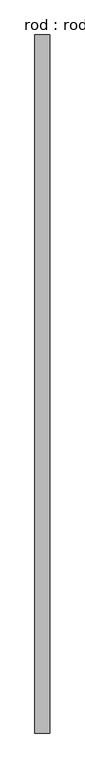
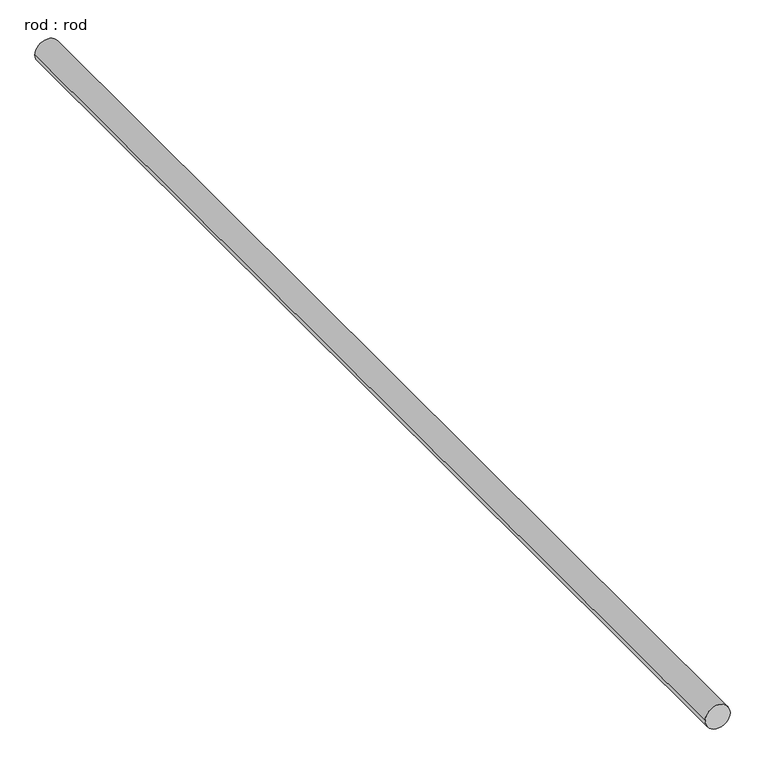
"""IFC4 building model written with IfcOpenShell, lengths in millimetres: proxy geometry, rod : rod."""

from ifc_helpers import new_model, si_unit, point, frame, frame_2d, origin, place, context, project, spatial, circle_curve, trimmed, segment, composite_curve, outline, extrude, source, transform, mapped, element, save


def rod_rod_8fb4618d(model_context):
    return source(origin(), model_context, "Body", "SweptSolid", [
        extrude(outline(composite_curve([segment(trimmed(circle_curve(frame_2d((0.0108462, 0.0)), 200.0), [point((0.0108462, 200.0))], [point((0.0108462, -200.0))], False, "CARTESIAN"), True, "CONTINUOUS"), segment(trimmed(circle_curve(frame_2d((0.0108462, 0.0)), 200.0), [point((0.0108462, -200.0))], [point((0.0108462, 200.0))], False, "CARTESIAN"), True, "CONTINUOUS")], self_intersect=False)), frame((0.0, -5228.6999561, 0.0), z_axis=(0.0, 1.0, 0.0), x_axis=(0.0, 0.0, 1.0)), (0.0, 0.0, 1.0), 18642.8571429),
    ])


if __name__ == "__main__":
    model = new_model("IFC4")
    model_context = context("Model", 3, world=origin())
    ifc_project = project(units=[si_unit("LENGTHUNIT", "METRE", prefix="MILLI")], contexts=[model_context])
    site = spatial("IfcSite", under=ifc_project)
    building = spatial("IfcBuilding", under=site)
    placement = place(None, origin())
    rod_rod_shape = rod_rod_8fb4618d(model_context)
    element("IfcBuildingElementProxy", 1, Name="rod : rod", ObjectType="rod : rod", at=placement, inside=building, context=model_context, shape_type="MappedRepresentation", body=[
        mapped(rod_rod_shape, transform((0.0, 0.0, 0.0), x_axis=(1.0, 0.0, 0.0), y_axis=(0.0, 1.0, 0.0), z_axis=(0.0, 0.0, 1.0))),
    ])
    save(model, "model.ifc")

# Revit data of these elements
# Type "rod : rod"
#   Default Elevation = 0
